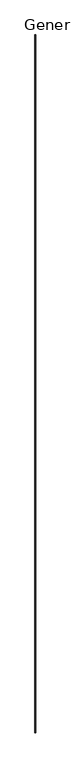
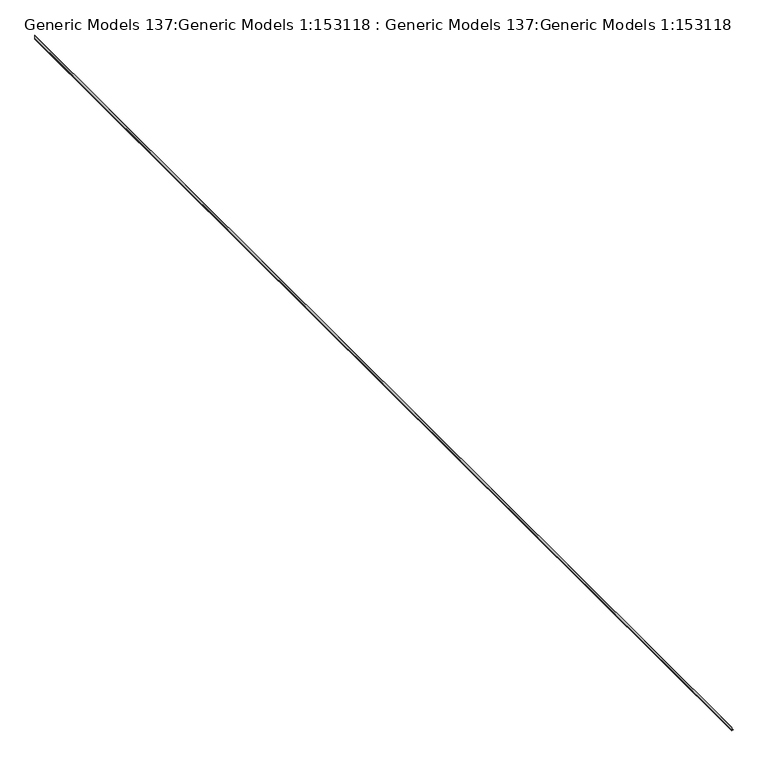
"""IFC4 building model written with IfcOpenShell, lengths in millimetres: proxy geometry, Generic Models 137:Generic Models 1:153118 : Generic Models 137:Generic Models 1:153118."""

from ifc_helpers import new_model, si_unit, frame, origin, place, context, project, spatial, polyline, outline, extrude, source, transform, mapped, element, save


def generic_models_137_generic_models_1_153118_generic_models_34c1130e(model_context):
    return source(origin(), model_context, "Body", "SweptSolid", [
        extrude(outline(polyline([(3654.4989461, 7240.9495965), (3660.9768942, 7261.1032131), (3667.7124299, 7240.1482131), (3711.7768942, 7240.1482131), (3711.7768942, 7238.8782131), (3666.7866506, 7238.8782131), (3660.9768942, 7256.9530108), (3655.4767363, 7239.8414082), (3650.3619859, 7238.8782131), (3650.1269543, 7240.1262756), (3654.4989461, 7240.9495965)])), frame((0.0, -6877.9974793, 0.0), z_axis=(0.0, 1.0, 0.0), x_axis=(0.0, 0.0, 1.0)), (0.0, 0.0, 1.0), 19050.0),
    ])


if __name__ == "__main__":
    model = new_model("IFC4")
    model_context = context("Model", 3, world=origin())
    ifc_project = project(units=[si_unit("LENGTHUNIT", "METRE", prefix="MILLI")], contexts=[model_context])
    site = spatial("IfcSite", under=ifc_project)
    building = spatial("IfcBuilding", under=site)
    placement = place(None, origin())
    generic_models_137_generic_models_1_153118_generic_models_shape = generic_models_137_generic_models_1_153118_generic_models_34c1130e(model_context)
    element("IfcBuildingElementProxy", 1, Name="Generic Models 137:Generic Models 1:153118 : Generic Models 137:Generic Models 1:153118", ObjectType="Generic Models 137:Generic Models 1:153118 : Generic Models 137:Generic Models 1:153118", at=placement, inside=building, context=model_context, shape_type="MappedRepresentation", body=[
        mapped(generic_models_137_generic_models_1_153118_generic_models_shape, transform((0.0, 0.0, 0.0), x_axis=(1.0, 0.0, 0.0), y_axis=(0.0, 1.0, 0.0), z_axis=(0.0, 0.0, 1.0))),
    ])
    save(model, "model.ifc")

# Revit data of these elements
# Type "Generic Models 137:Generic Models 1:153118 : Generic Models 137:Generic Models 1:153118"
#   NameOverride = "Generic Models 137:Generic Models 1:153118"
#   ObjectTypeOverride = "Generic Models 137:Generic Models 1"
#   Reference = "Generic Models 1"
#   Category = "Generic Models"
#   Tag = "153118"
# Element 1 (IfcBuildingElementProxy, "Generic Models 137:Generic Models 1:153118 : Generic Models 137:Generic Models 1:153118")
#   Materials on its faces: "_16 GA. COPPER WEEP SCREED W/ MIN. 3 1/2\" ATTACHEMENT FLANGE - LAP UNDERLAYMENT OVER WEED SCREED 3430"
# Materials
#   "_16 GA. COPPER WEEP SCREED W/ MIN. 3 1/2\" ATTACHEMENT FLANGE - LAP UNDERLAYMENT OVER WEED SCREED 3430": class "Unassigned", colour RGB 253 192 103, transparency 0
